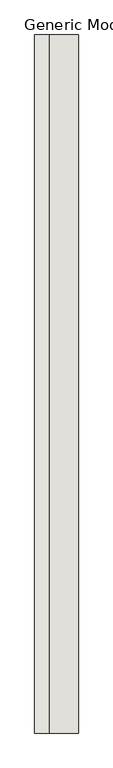
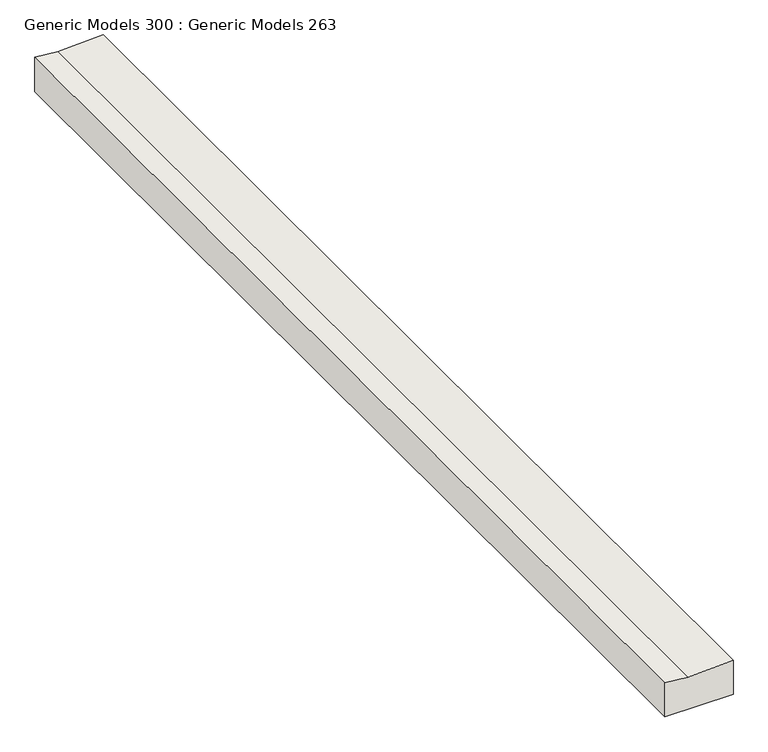
"""IFC4 building model written with IfcOpenShell, lengths in millimetres: wall geometry, Generic Models 300 : Generic Models 263."""

from ifc_helpers import new_model, si_unit, frame, origin, place, context, project, spatial, polyline, outline, extrude, source, transform, mapped, element, save


def generic_models_300_generic_models_263_12a764e5(model_context):
    return source(origin(), model_context, "Body", "SweptSolid", [
        extrude(outline(polyline([(-139.1379392, 91579.9797726), (-381.0, 91579.9797726), (-381.0, 92037.1797726), (-139.7, 92037.1797726), (-152.4, 91732.3797726), (-139.1379392, 91579.9797726)])), frame((0.0, -6732.6272578, 0.0), z_axis=(0.0, 1.0, 0.0), x_axis=(0.0, 0.0, 1.0)), (0.0, 0.0, 1.0), 7315.2),
    ])


if __name__ == "__main__":
    model = new_model("IFC4")
    model_context = context("Model", 3, world=origin())
    ifc_project = project(units=[si_unit("LENGTHUNIT", "METRE", prefix="MILLI")], contexts=[model_context])
    site = spatial("IfcSite", under=ifc_project)
    building = spatial("IfcBuilding", under=site)
    placement = place(None, origin())
    generic_models_300_generic_models_263_shape = generic_models_300_generic_models_263_12a764e5(model_context)
    element("IfcWall", 1, ObjectType="Generic Models 300 : Generic Models 263", at=placement, inside=building, context=model_context, shape_type="MappedRepresentation", body=[
        mapped(generic_models_300_generic_models_263_shape, transform((0.0, 0.0, 0.0), x_axis=(1.0, 0.0, 0.0), y_axis=(0.0, 1.0, 0.0), z_axis=(0.0, 0.0, 1.0))),
    ])
    save(model, "model.ifc")

# Revit data of these elements
# Element 1 (IfcWall, "Generic Models 300 : Generic Models 263")
#   Materials on its faces: "CONCRETE CURB"
# Materials
#   "CONCRETE CURB": class "Concrete", colour RGB 191 191 191, transparency 0, Description = "Cast-in-place concrete", Cost = 0
